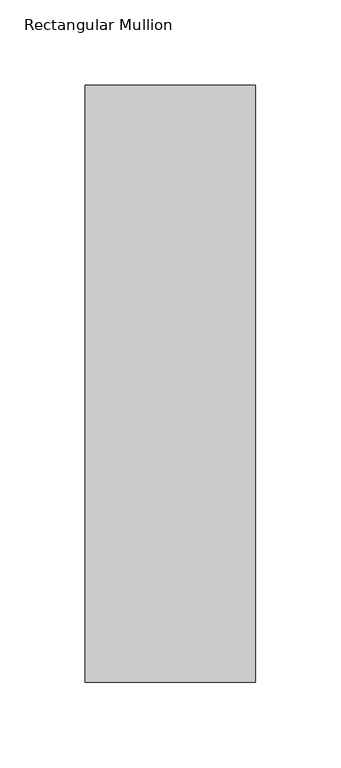
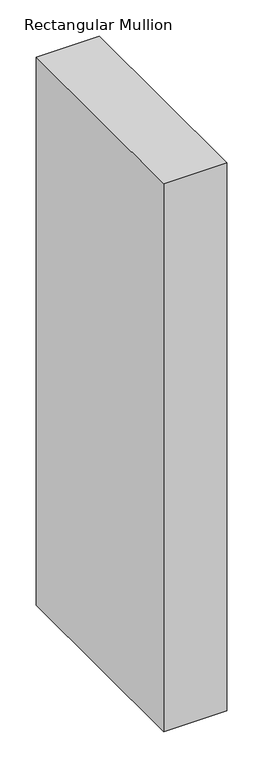
"""IFC4 building model written with IfcOpenShell, lengths in millimetres: member geometry, Rectangular Mullion : WWm-100x350-100mmOffset."""

from ifc_helpers import new_model, si_unit, frame, origin, place, context, project, spatial, polyline, outline, extrude, source, transform, mapped, element, save


def rectangular_mullion_5d092932(model_context):
    return source(origin(), model_context, "Body", "SweptSolid", [
        extrude(outline(polyline([(0.0, 175.0), (0.0, -175.0), (-100.0, -175.0), (-100.0, 175.0), (0.0, 175.0)])), frame((0.0, 0.0, -920.0), z_axis=(0.0, 0.0, 1.0), x_axis=(1.0, 0.0, 0.0)), (0.0, 0.0, 1.0), 920.0),
    ])


if __name__ == "__main__":
    model = new_model("IFC4")
    model_context = context("Model", 3, world=origin())
    ifc_project = project(units=[si_unit("LENGTHUNIT", "METRE", prefix="MILLI")], contexts=[model_context])
    site = spatial("IfcSite", under=ifc_project)
    building = spatial("IfcBuilding", under=site)
    placement = place(None, origin())
    rectangular_mullion_shape = rectangular_mullion_5d092932(model_context)
    element("IfcMember", 1, ObjectType="Rectangular Mullion : WWm-100x350-100mmOffset", at=placement, inside=building, context=model_context, shape_type="MappedRepresentation", body=[
        mapped(rectangular_mullion_shape, transform((0.0, 0.0, 0.0), x_axis=(1.0, 0.0, 0.0), y_axis=(0.0, 1.0, 0.0), z_axis=(0.0, 0.0, 1.0))),
    ])
    save(model, "model.ifc")

# Revit data of these elements
# Type "Rectangular Mullion : WWm-100x350-100mmOffset"
#   built-in parameter 1007304 = 1.14829 (stored number, unit not read)
#   built-in parameter 1007301 = 0.164042 (stored number, unit not read)
#   built-in parameter 1007300 = 0.164042 (stored number, unit not read)
# Element 1 (IfcMember, "Rectangular Mullion : WWm-100x350-100mmOffset")
#   Materials on its faces: "WW-EC-RGB-Mullion"
# Materials
#   "WW-EC-RGB-Mullion": class "Generic", colour RGB 255 255 255, transparency 0, Comments = "If region requests black mullions, switch asset color to RGB 25-25-25", Description = "Generic Color", Cost = 0
